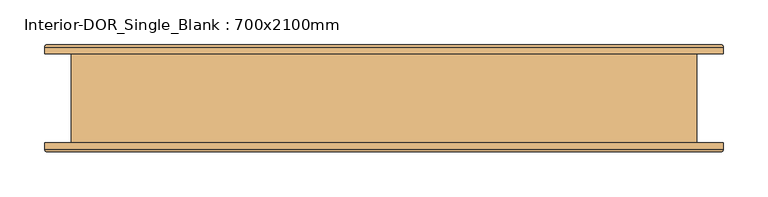
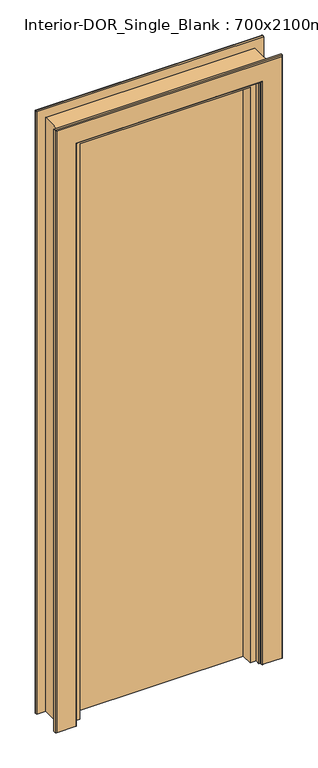
"""IFC4 building model written with IfcOpenShell, lengths in millimetres: door geometry, Interior-DOR_Single_Blank : 700x2100mm."""

from ifc_helpers import new_model, si_unit, frame, origin, origin_with_axes, place, context, project, spatial, polyline, circle_curve, ellipse_curve, outline, extrude, faceted_brep, source, transform, mapped, element, save
from ifc_brep_helpers import plane_surface, cylinder_surface, advanced_brep


def interior_dor_single_blank_700x2100mm_59f542ac(model_context):
    return source(origin(), model_context, "Body", "SolidModel", [
        advanced_brep(
        [(-310.0, 50.0, 0.0), (-380.0, 50.0, 0.0), (-380.0, 57.0, 0.0), (-377.0, 60.0, 0.0), (-313.0, 60.0, 0.0), (-310.0, 57.0, 0.0), (-310.0, 57.0, 2060.0), (-310.0, 50.0, 2060.0), (-313.0, 60.0, 2063.0), (-377.0, 60.0, 2127.0), (377.0, 60.0, 2127.0), (377.0, 60.0, 0.0), (313.0, 60.0, 0.0), (313.0, 60.0, 2063.0), (-380.0, 57.0, 2130.0), (-380.0, 50.0, 2130.0), (310.0, 50.0, 2060.0), (310.0, 50.0, 0.0), (380.0, 50.0, 0.0), (380.0, 50.0, 2130.0), (310.0, 57.0, 0.0), (310.0, 57.0, 2060.0), (380.0, 57.0, 0.0), (380.0, 57.0, 2130.0)],
        [
            (0, 1),
            (1, 2),
            (2, 3, circle_curve(frame((-377.0, 57.0, 0.0), z_axis=(0.0, 0.0, -1.0), x_axis=(-1.0, 0.0, 0.0)), 3.0)),
            (3, 4),
            (4, 5, circle_curve(frame((-313.0, 57.0, 0.0), z_axis=(0.0, 0.0, -1.0), x_axis=(-1.0, 0.0, 0.0)), 3.0)),
            (5, 0),
            (5, 6),
            (6, 7),
            (7, 0),
            (4, 8),
            (8, 6, ellipse_curve(frame((-313.0, 57.0, 2063.0), z_axis=(-0.7071067811865475, 0.0, -0.7071067811865475), x_axis=(0.7071067811865474, 0.0, -0.7071067811865476)), 4.2426407, 3.0)),
            (3, 9),
            (9, 10),
            (10, 11),
            (11, 12),
            (12, 13),
            (13, 8),
            (2, 14),
            (14, 9, ellipse_curve(frame((-377.0, 57.0, 2127.0), z_axis=(-0.7071067811865475, 0.0, -0.7071067811865475), x_axis=(0.7071067811865474, 0.0, -0.7071067811865476)), 4.2426407, 3.0)),
            (1, 15),
            (15, 14),
            (7, 16),
            (16, 17),
            (17, 18),
            (18, 19),
            (19, 15),
            (12, 20, circle_curve(frame((313.0, 57.0, 0.0), z_axis=(0.0, 0.0, 1.0), x_axis=(1.0, 0.0, 0.0)), 3.0)),
            (20, 21),
            (21, 13, ellipse_curve(frame((313.0, 57.0, 2063.0), z_axis=(0.7071067811865475, 0.0, -0.7071067811865475), x_axis=(0.7071067811865474, 0.0, 0.7071067811865476)), 4.2426407, 3.0)),
            (17, 20),
            (11, 22, circle_curve(frame((377.0, 57.0, 0.0), z_axis=(0.0, 0.0, -1.0), x_axis=(1.0, 0.0, 0.0)), 3.0)),
            (22, 18),
            (23, 22),
            (10, 23, ellipse_curve(frame((377.0, 57.0, 2127.0), z_axis=(0.7071067811865475, 0.0, -0.7071067811865475), x_axis=(0.7071067811865474, 0.0, 0.7071067811865476)), 4.2426407, 3.0)),
            (23, 19),
            (16, 21),
            (6, 21),
            (14, 23),
        ],
        [
            plane_surface(frame((-350.0, -50.0, 0.0), z_axis=(0.0, 0.0, -1.0), x_axis=(0.0, 1.0, 0.0))),
            plane_surface(frame((-310.0, 50.0, 0.0), z_axis=(1.0, 0.0, 0.0), x_axis=(0.0, 0.0, 1.0))),
            cylinder_surface(frame((-313.0, 57.0, 0.0), z_axis=(0.0, 0.0, -1.0), x_axis=(-1.0, 0.0, 0.0)), 3.0),
            plane_surface(frame((-313.0, 60.0, 0.0), z_axis=(0.0, 1.0, 0.0), x_axis=(0.0, 0.0, 1.0))),
            cylinder_surface(frame((-377.0, 57.0, 0.0), z_axis=(0.0, 0.0, -1.0), x_axis=(-1.0, 0.0, 0.0)), 3.0),
            plane_surface(frame((-380.0, 57.0, 0.0), z_axis=(-1.0, 0.0, 0.0), x_axis=(0.0, 0.0, 1.0))),
            plane_surface(frame((-380.0, 50.0, 0.0), z_axis=(0.0, -1.0, 0.0), x_axis=(0.0, 0.0, 1.0))),
            cylinder_surface(frame((313.0, 57.0, 2100.0), z_axis=(0.0, 0.0, 1.0), x_axis=(1.0, 0.0, 0.0)), 3.0),
            plane_surface(frame((350.0, -50.0, 0.0), z_axis=(0.0, 0.0, -1.0), x_axis=(0.0, 1.0, 0.0))),
            cylinder_surface(frame((377.0, 57.0, 2100.0), z_axis=(0.0, 0.0, 1.0), x_axis=(1.0, 0.0, 0.0)), 3.0),
            plane_surface(frame((380.0, 57.0, 2130.0), z_axis=(1.0, 0.0, 0.0), x_axis=(0.0, 0.0, -1.0))),
            plane_surface(frame((310.0, 50.0, 2060.0), z_axis=(-1.0, 0.0, 0.0), x_axis=(0.0, 0.0, -1.0))),
            plane_surface(frame((-310.0, 50.0, 2060.0), z_axis=(0.0, 0.0, -1.0), x_axis=(1.0, 0.0, 0.0))),
            cylinder_surface(frame((-350.0, 57.0, 2063.0), z_axis=(-1.0, 0.0, 0.0), x_axis=(0.0, 0.0, 1.0)), 3.0),
            cylinder_surface(frame((-350.0, 57.0, 2127.0), z_axis=(-1.0, 0.0, 0.0), x_axis=(0.0, 0.0, 1.0)), 3.0),
            plane_surface(frame((-380.0, 57.0, 2130.0), z_axis=(0.0, 0.0, 1.0), x_axis=(1.0, 0.0, 0.0))),
        ],
        [
            (0, [[1, 2, 3, 4, 5, 6]]),
            (1, [[7, 8, 9, -6]]),
            (2, [[10, 11, -7, -5]]),
            (3, [[12, 13, 14, 15, 16, 17, -10, -4]]),
            (4, [[18, 19, -12, -3]]),
            (5, [[20, 21, -18, -2]]),
            (6, [[-9, 22, 23, 24, 25, 26, -20, -1]]),
            (7, [[-16, 27, 28, 29]]),
            (8, [[30, -27, -15, 31, 32, -24]]),
            (9, [[33, -31, -14, 34]]),
            (10, [[-25, -32, -33, 35]]),
            (11, [[-28, -30, -23, 36]]),
            (12, [[37, -36, -22, -8]]),
            (13, [[-17, -29, -37, -11]]),
            (14, [[38, -34, -13, -19]]),
            (15, [[-26, -35, -38, -21]]),
        ],
    ),
        advanced_brep(
        [(-380.0, -50.0, 0.0), (-310.0, -50.0, 0.0), (-310.0, -57.0, 0.0), (-313.0, -60.0, 0.0), (-377.0, -60.0, 0.0), (-380.0, -57.0, 0.0), (-380.0, -57.0, 2130.0), (-380.0, -50.0, 2130.0), (-377.0, -60.0, 2127.0), (-313.0, -60.0, 2063.0), (313.0, -60.0, 2063.0), (313.0, -60.0, 0.0), (377.0, -60.0, 0.0), (377.0, -60.0, 2127.0), (-310.0, -57.0, 2060.0), (-310.0, -50.0, 2060.0), (380.0, -50.0, 2130.0), (380.0, -50.0, 0.0), (310.0, -50.0, 0.0), (310.0, -50.0, 2060.0), (380.0, -57.0, 0.0), (380.0, -57.0, 2130.0), (310.0, -57.0, 0.0), (310.0, -57.0, 2060.0)],
        [
            (0, 1),
            (1, 2),
            (2, 3, circle_curve(frame((-313.0, -57.0, 0.0), z_axis=(0.0, 0.0, -1.0), x_axis=(-1.0, 0.0, 0.0)), 3.0)),
            (3, 4),
            (4, 5, circle_curve(frame((-377.0, -57.0, 0.0), z_axis=(0.0, 0.0, -1.0), x_axis=(-1.0, 0.0, 0.0)), 3.0)),
            (5, 0),
            (5, 6),
            (6, 7),
            (7, 0),
            (4, 8),
            (8, 6, ellipse_curve(frame((-377.0, -57.0, 2127.0), z_axis=(-0.7071067811865475, 0.0, -0.7071067811865475), x_axis=(0.7071067811865474, 0.0, -0.7071067811865476)), 4.2426407, 3.0)),
            (3, 9),
            (9, 10),
            (10, 11),
            (11, 12),
            (12, 13),
            (13, 8),
            (2, 14),
            (14, 9, ellipse_curve(frame((-313.0, -57.0, 2063.0), z_axis=(-0.7071067811865475, 0.0, -0.7071067811865475), x_axis=(0.7071067811865474, 0.0, -0.7071067811865476)), 4.2426407, 3.0)),
            (1, 15),
            (15, 14),
            (7, 16),
            (16, 17),
            (17, 18),
            (18, 19),
            (19, 15),
            (12, 20, circle_curve(frame((377.0, -57.0, 0.0), z_axis=(0.0, 0.0, 1.0), x_axis=(1.0, 0.0, 0.0)), 3.0)),
            (20, 21),
            (21, 13, ellipse_curve(frame((377.0, -57.0, 2127.0), z_axis=(0.7071067811865475, 0.0, -0.7071067811865475), x_axis=(0.7071067811865474, 0.0, 0.7071067811865476)), 4.2426407, 3.0)),
            (17, 20),
            (11, 22, circle_curve(frame((313.0, -57.0, 0.0), z_axis=(0.0, 0.0, -1.0), x_axis=(1.0, 0.0, 0.0)), 3.0)),
            (22, 18),
            (23, 22),
            (10, 23, ellipse_curve(frame((313.0, -57.0, 2063.0), z_axis=(0.7071067811865475, 0.0, -0.7071067811865475), x_axis=(0.7071067811865474, 0.0, 0.7071067811865476)), 4.2426407, 3.0)),
            (23, 19),
            (16, 21),
            (6, 21),
            (14, 23),
        ],
        [
            plane_surface(frame((-350.0, -50.0, 0.0), z_axis=(0.0, 0.0, -1.0), x_axis=(0.0, 1.0, 0.0))),
            plane_surface(frame((-380.0, -50.0, 0.0), z_axis=(-1.0, 0.0, 0.0), x_axis=(0.0, 0.0, 1.0))),
            cylinder_surface(frame((-377.0, -57.0, 0.0), z_axis=(0.0, 0.0, -1.0), x_axis=(-1.0, 0.0, 0.0)), 3.0),
            plane_surface(frame((-377.0, -60.0, 0.0), z_axis=(0.0, -1.0, 0.0), x_axis=(0.0, 0.0, 1.0))),
            cylinder_surface(frame((-313.0, -57.0, 0.0), z_axis=(0.0, 0.0, -1.0), x_axis=(-1.0, 0.0, 0.0)), 3.0),
            plane_surface(frame((-310.0, -57.0, 0.0), z_axis=(1.0, 0.0, 0.0), x_axis=(0.0, 0.0, 1.0))),
            plane_surface(frame((-310.0, -50.0, 0.0), z_axis=(0.0, 1.0, 0.0), x_axis=(0.0, 0.0, 1.0))),
            cylinder_surface(frame((377.0, -57.0, 2100.0), z_axis=(0.0, 0.0, 1.0), x_axis=(1.0, 0.0, 0.0)), 3.0),
            plane_surface(frame((350.0, -50.0, 0.0), z_axis=(0.0, 0.0, -1.0), x_axis=(0.0, 1.0, 0.0))),
            cylinder_surface(frame((313.0, -57.0, 2100.0), z_axis=(0.0, 0.0, 1.0), x_axis=(1.0, 0.0, 0.0)), 3.0),
            plane_surface(frame((310.0, -57.0, 2060.0), z_axis=(-1.0, 0.0, 0.0), x_axis=(0.0, 0.0, -1.0))),
            plane_surface(frame((380.0, -50.0, 2130.0), z_axis=(1.0, 0.0, 0.0), x_axis=(0.0, 0.0, -1.0))),
            plane_surface(frame((-380.0, -50.0, 2130.0), z_axis=(0.0, 0.0, 1.0), x_axis=(1.0, 0.0, 0.0))),
            cylinder_surface(frame((-350.0, -57.0, 2127.0), z_axis=(-1.0, 0.0, 0.0), x_axis=(0.0, 0.0, 1.0)), 3.0),
            cylinder_surface(frame((-350.0, -57.0, 2063.0), z_axis=(-1.0, 0.0, 0.0), x_axis=(0.0, 0.0, 1.0)), 3.0),
            plane_surface(frame((-310.0, -57.0, 2060.0), z_axis=(0.0, 0.0, -1.0), x_axis=(1.0, 0.0, 0.0))),
        ],
        [
            (0, [[1, 2, 3, 4, 5, 6]]),
            (1, [[7, 8, 9, -6]]),
            (2, [[10, 11, -7, -5]]),
            (3, [[12, 13, 14, 15, 16, 17, -10, -4]]),
            (4, [[18, 19, -12, -3]]),
            (5, [[20, 21, -18, -2]]),
            (6, [[-9, 22, 23, 24, 25, 26, -20, -1]]),
            (7, [[-16, 27, 28, 29]]),
            (8, [[30, -27, -15, 31, 32, -24]]),
            (9, [[33, -31, -14, 34]]),
            (10, [[-25, -32, -33, 35]]),
            (11, [[-28, -30, -23, 36]]),
            (12, [[37, -36, -22, -8]]),
            (13, [[-17, -29, -37, -11]]),
            (14, [[38, -34, -13, -19]]),
            (15, [[-26, -35, -38, -21]]),
        ],
    ),
        faceted_brep([(-350.0, -50.0, 0.0), (-350.0, 50.0, 0.0), (-305.0, 50.0, 0.0), (-305.0, 5.0, 0.0), (-285.0, 5.0, 0.0), (-285.0, -35.0, 0.0), (-305.0, -35.0, 0.0), (-305.0, -50.0, 0.0), (-305.0, -50.0, 2055.0), (305.0, -50.0, 2055.0), (305.0, -50.0, 0.0), (350.0, -50.0, 0.0), (350.0, -50.0, 2100.0), (-350.0, -50.0, 2100.0), (-305.0, -35.0, 2055.0), (-285.0, -35.0, 2035.0), (285.0, -35.0, 2035.0), (285.0, -35.0, 0.0), (305.0, -35.0, 0.0), (305.0, -35.0, 2055.0), (-285.0, 5.0, 2035.0), (-305.0, 5.0, 2055.0), (305.0, 5.0, 2055.0), (305.0, 5.0, 0.0), (285.0, 5.0, 0.0), (285.0, 5.0, 2035.0), (-305.0, 50.0, 2055.0), (-350.0, 50.0, 2100.0), (350.0, 50.0, 2100.0), (350.0, 50.0, 0.0), (305.0, 50.0, 0.0), (305.0, 50.0, 2055.0)], [[[0, 1, 2, 3, 4, 5, 6, 7]], [[7, 8, 9, 10, 11, 12, 13, 0]], [[6, 14, 8, 7]], [[5, 15, 16, 17, 18, 19, 14, 6]], [[4, 20, 15, 5]], [[3, 21, 22, 23, 24, 25, 20, 4]], [[2, 26, 21, 3]], [[1, 27, 28, 29, 30, 31, 26, 2]], [[0, 13, 27, 1]], [[12, 11, 29, 28]], [[11, 10, 18, 17, 24, 23, 30, 29]], [[19, 18, 10, 9]], [[25, 24, 17, 16]], [[31, 30, 23, 22]], [[20, 25, 16, 15]], [[26, 31, 22, 21]], [[13, 12, 28, 27]], [[14, 19, 9, 8]]]),
        extrude(outline(polyline([(305.0, 50.0), (305.0, 5.0), (-305.0, 5.0), (-305.0, 50.0), (305.0, 50.0)])), origin_with_axes(), (0.0, 0.0, 1.0), 2055.0),
    ])


if __name__ == "__main__":
    model = new_model("IFC4")
    model_context = context("Model", 3, world=origin())
    ifc_project = project(units=[si_unit("LENGTHUNIT", "METRE", prefix="MILLI")], contexts=[model_context])
    site = spatial("IfcSite", under=ifc_project)
    building = spatial("IfcBuilding", under=site)
    placement = place(None, origin())
    interior_dor_single_blank_700x2100mm_shape = interior_dor_single_blank_700x2100mm_59f542ac(model_context)
    element("IfcDoor", 1, ObjectType="Interior-DOR_Single_Blank : 700x2100mm", at=placement, inside=building, context=model_context, shape_type="MappedRepresentation", body=[
        mapped(interior_dor_single_blank_700x2100mm_shape, transform((0.0, 0.0, 0.0), x_axis=(1.0, 0.0, 0.0), y_axis=(0.0, 1.0, 0.0), z_axis=(0.0, 0.0, 1.0))),
    ])
    save(model, "model.ifc")

# Revit data of these elements
# Type "Interior-DOR_Single_Blank : 700x2100mm"
#   Type IfcGUID = "1sWU2cMPP4xwRoAc3TXQKN"
#   Assembly Code = "C1020120"
#   Type Mark = "196"
#   Classification.Uniclass.EF.Number = "EF_25_30"
#   Classification.Uniclass.EF.Description = "Doors and windows"
#   WindLoadRating = "n/a"
#   WaterTightnessRating = "n/a"
#   WarrantyStartDate [instance default] = "1900-12-31T23:59:59"
#   WarrantyGuarantorParts = "n/a"
#   WarrantyGuarantorLabor = "n/a"
#   WarrantyDurationUnit = "year"
#   WarrantyDurationParts = "n/a"
#   WarrantyDurationLabor = "n/a"
#   WarrantyDescription = "n/a"
#   Version = "2"
#   Uniclass2015Version = "Systems v1.9"
#   Uniclass2015Title = "Doorset systems"
#   Uniclass2015Code = "Ss_25_30_20_25"
#   URL = "www.nationalbimlibrary.com"
#   TagNumber [instance default] = "n/a"
#   SustainabilityPerformance = "n/a"
#   Status = "UNSET"
#   Size = "1010 x 2100 mm"
#   Shape = "n/a"
#   SerialNumber [instance default] = "n/a"
#   SecurityRating = "n/a"
#   Revision = "n/a"
#   ReplacementCost = "n/a"
#   Reference = "n/a"
#   ProductInformation = "n/a"
#   Operation = "SINGLE_SWING_RIGHT"
#   OmniClassVersion = "Table 22 2012-05-16"
#   OmniClassTitle = "Doors and Frames"
#   OmniClassCode = "22-08 10 00"
#   Name = "DoorsetSystem_Interior-Single_Blank"
#   NBSReference = "25-50-20/120"
#   NBSDescription = "Doorset system"
#   NBSCertification = "www.nationalbimlibrary.com/cert/mlf45nxc"
#   ModelReference = "Interior Single Door"
#   ModelNumber = "n/a"
#   Model = "Interior Single Door"
#   MechanicalLoadRating = "n/a"
#   Material = "n/a"
#   ManufacturerURL = "n/a"
#   ManufacturerName = "n/a"
#   Manufacturer = "info@theNBS.com"
#   InstallationDate [instance default] = "1900-12-31T23:59:59"
#   IfcExportType = "DOOR"
#   IfcExportAs = "IfcDoorType"
#   HygrothermalRating = "n/a"
#   Grade = "n/a"
#   FireRating = "n/a"
#   Fire Rating = "n/a"
#   Finish = "n/a"
#   Features = "n/a"
#   ExpectedLife = "n/a"
#   DurationUnit = "n/a"
#   DurabilityRating = "n/a"
#   DoorNumber [instance default] = "n/a"
#   Description = "Generic single interior door"
#   Construction Type = "USERDEFINED"
#   Constituents = "n/a"
#   ComponentNumber [instance default] = "n/a"
#   Color = "n/a"
#   CodePerformance = "n/a"
#   Category = "Ss_25_30_20_25:Doorset systems"
#   BarCode [instance default] = "n/a"
#   BIMObjectName = "NBS_DoorsetSystem_Interior-Single_Blank"
#   Author = "NBS"
#   AssetType = "Fixed"
#   AssetIdentifier [instance default] = "n/a"
#   AcousticRating = "n/a"
#   AccessibilityPerformance = "n/a"
#   Width = 0.7 m
#   WallThickness [instance default] = 0.15 m
#   ThresholdHeight = 0.015 m
#   Thickness = 0.15 m
#   ThermalTransmittance = 0
#   StructuralToleranceJamb = 0 m
#   StructuralToleranceHead = 0 m
#   StructuralOpeningWidth = 0.7 m
#   StructuralOpeningHeight = 2.1 m
#   StopProjection = 0.02 m
#   StopDepth = 0.04 m
#   Rough Width [instance default] = 0.7 m
#   Rough Height [instance default] = 2.1 m
#   RebateDepth = 0.045 m
#   PanelWidth = 0.61 m
#   PanelUndercut = 0 m
#   PanelHeight = 2.055 m
#   PanelDepth = 0.045 m
#   OpeningTolerance = 0 m
#   NominalWidth = 0.7 m
#   NominalLength = 0 m
#   NominalHeight = 2.1 m
#   Infiltration = 0
#   Height = 2.1 m
#   GlazingAreaFraction = 0
#   FrameThickness = 0.045 m
#   FrameSetback [instance default] = 0 m
#   FrameDepth [instance default] = 0.15 m
#   FinishThicknessInternal [instance default] = 0 m
#   FinishThicknessExternal [instance default] = 0 m
#   ClearOpeningWidth = 0.57 m
#   ClearOpeningHeight = 2.035 m
#   CalculatedInteriorVoidDepth [instance default] = 0.3 m
#   ArchitraveWidth = 0.07 m
#   ArchitraveThickness = 0.01 m
#   ArchitraveSetbackFromFrameFace = 0.005 m
#   SmokeStop = no
#   SingleRebate = no
#   SelfClosing = no
#   PlantedStop = yes
#   IsExternal = no
#   HasDrive = no
#   HandicapAccessible = no
#   Wall Closure = 4
#   FireExit = no
#   ArchitraveFrontRequired [instance default] = yes
#   ArchitraveBackRequired [instance default] = yes
#   PanelMaterial = NBS_Concept
#   HardwareFinish = NBS_Concept
#   FrameSectionMaterial = NBS_Concept
#   Function = (empty or 0)
#   Cost = 0
# Element 1 (IfcDoor, "Interior-DOR_Single_Blank : 700x2100mm")
#   WallThickness = 0.1 m
#   FrameDepth = 0.1 m
#   Materials on its faces: "NBS_Concept"
# Materials
#   "NBS_Concept": class "Generic", colour RGB 255 255 255, transparency 0, Description = "To be specified", Cost = 0
